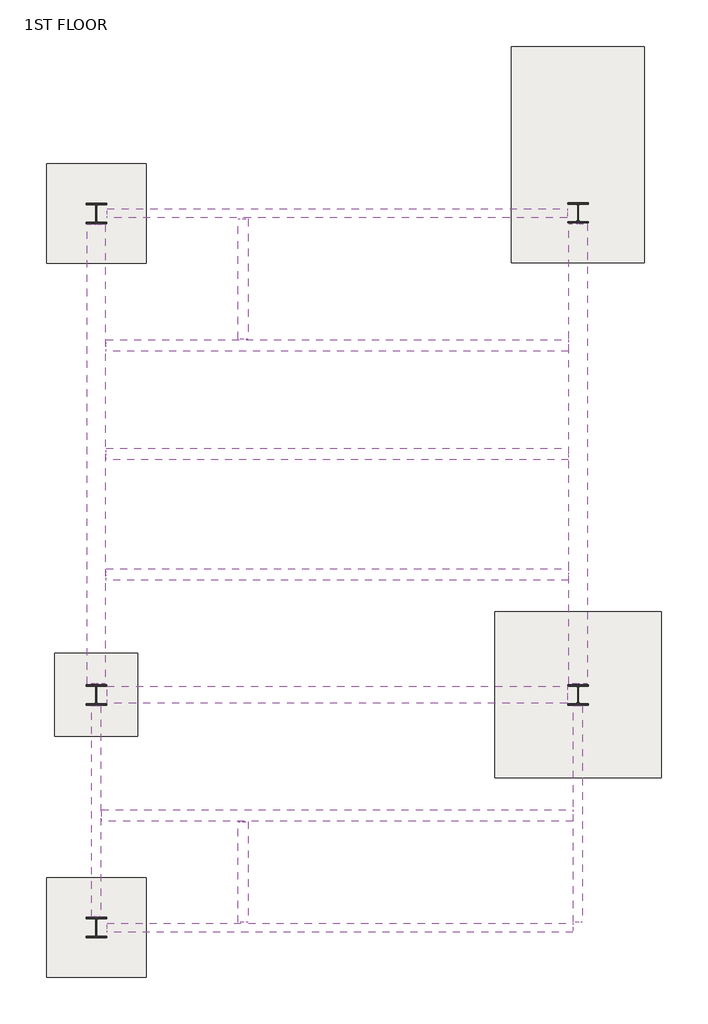
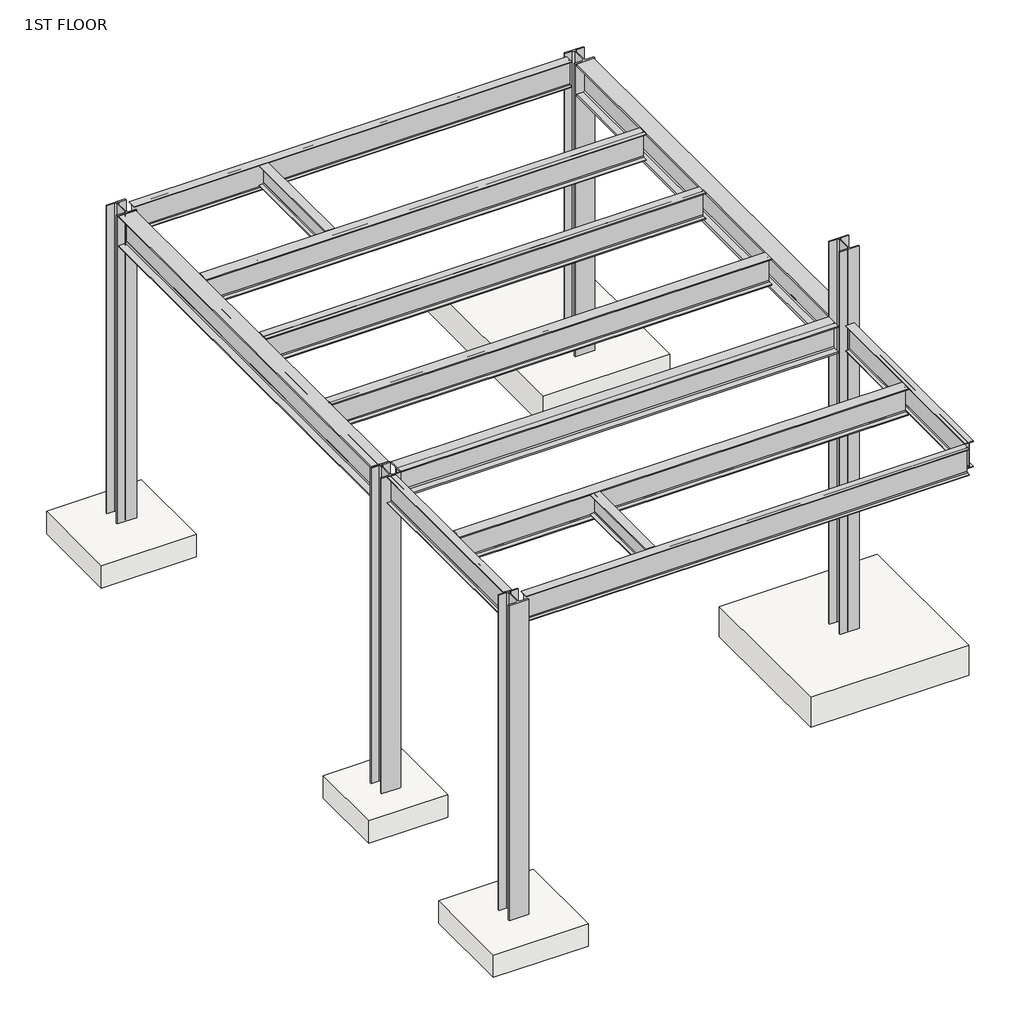
# One storey: 13 beams, 5 columns, 5 slabs.
# Revit data of these elements (continued)
# Element 16 (IfcColumn, "W-Wide Flange-Column : W14X132") (continued)
#   RS Unique Id = 265123
#   Column Material = Metal - Steel - ASTM A992
#   Phase Created = New Construction
#   Materials on its faces: "Metal - Steel - ASTM A992"
# Element 17 (IfcColumn, "W-Wide Flange-Column : W14X132")
#   RM User Number = 299
#   RM Unique Id = 4749
#   RS Unique Id = 265145
#   Column Material = Metal - Steel - ASTM A992
#   Phase Created = New Construction
#   Materials on its faces: "Metal - Steel - ASTM A992"
# Element 18 (IfcColumn, "W-Wide Flange-Column : W14X132")
#   RM User Number = 35
#   RM Unique Id = 4525
#   RS Unique Id = 247418
#   Column Material = Metal - Steel - ASTM A992
#   Phase Created = New Construction
#   Materials on its faces: "Metal - Steel - ASTM A992"
# Element 19 (IfcSlab, "Footing-Rectangular : 6'-0\" x 6''-0\"")
#   RM User Number = 0
#   RM Unique Id = 0
#   RS Unique Id = 268534
#   Footing Material = Concrete - Cast-in-Place Concrete
#   Phase Created = New Construction
#   Materials on its faces: "Concrete - Cast-in-Place Concrete"
# Element 20 (IfcSlab, "Footing-Rectangular : 6'-0\" x 6''-0\"")
#   RM User Number = 0
#   RM Unique Id = 0
#   RS Unique Id = 268536
#   Footing Material = Concrete - Cast-in-Place Concrete
#   Phase Created = New Construction
#   Materials on its faces: "Concrete - Cast-in-Place Concrete"
# Element 21 (IfcSlab, "Footing-Rectangular : 8''-0\" x 13'-0\"")
#   RM User Number = 0
#   RM Unique Id = 0
#   RS Unique Id = 344702
#   Footing Material = Concrete - Cast-in-Place Concrete
#   Phase Created = New Construction
#   Materials on its faces: "Concrete - Cast-in-Place Concrete"
# Element 22 (IfcSlab, "Footing-Rectangular : 10-0' x 10'-0\"")
#   RM User Number = 0
#   RM Unique Id = 0
#   RS Unique Id = 250894
#   Footing Material = Concrete - Cast-in-Place Concrete
#   Phase Created = New Construction
#   Materials on its faces: "Concrete - Cast-in-Place Concrete"
# Element 23 (IfcSlab, "Footing-Rectangular : 5'-0\" x 5'-0\"")
#   RM User Number = 0
#   RM Unique Id = 0
#   RS Unique Id = 268535
#   Footing Material = Concrete - Cast-in-Place Concrete
#   Phase Created = New Construction
#   Materials on its faces: "Concrete - Cast-in-Place Concrete"
# Materials
#   "Metal - Steel - ASTM A992": class "Metal", colour RGB 128 0 0, transparency 0
#   "Concrete - Cast-in-Place Concrete": class "Concrete", colour RGB 192 192 192, transparency 0.4
